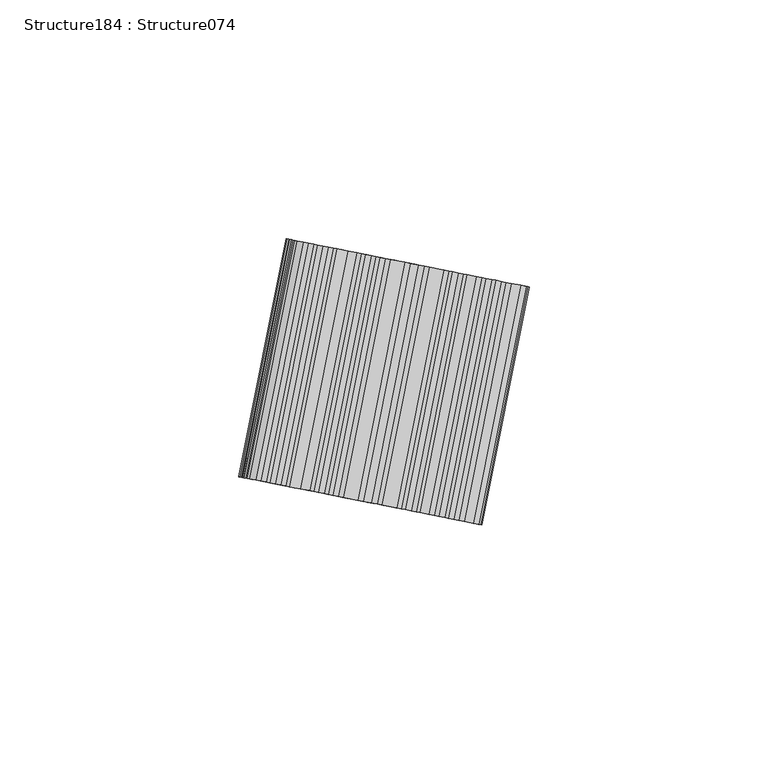
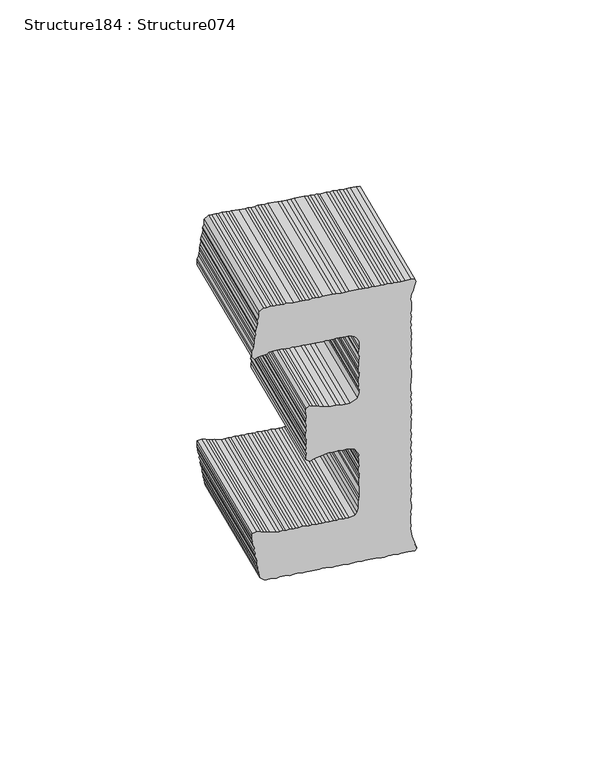
"""IFC4 building model written with IfcOpenShell, lengths in millimetres: proxy geometry, Structure184 : Structure074."""

import ifcopenshell
import ifcopenshell.guid

model = None  # the IFC model being written
_history = None  # IfcOwnerHistory: only IFC2X3 demands one
_inside = {}  # id of a spatial element -> (the spatial element, [elements in it])
_under = {}  # id of a project, library or spatial element -> (it, [spatial elements below it])
_declared = {}  # id of a project -> (the project, [libraries it declares])
_typed = {}  # id of a type object -> (the type object, [elements of that type])
_made_of = {}  # id of a material, layer set ... -> (it, [elements and type objects made of it])


def new_model(schema):
    """Start an empty IFC model of exactly this schema.

    Asked for "IFC4X3", IfcOpenShell would pick the latest addendum, in which some entities
    have other attributes; the version numbers below select the first issue.
    IFC2X3 requires an IfcOwnerHistory on every rooted entity: one is made here for all.
    """
    global model, _history
    if schema == "IFC4X3":
        model = ifcopenshell.file(schema_version=(4, 3, 0, 0))
    else:
        model = ifcopenshell.file(schema=schema)
    _inside.clear()
    _under.clear()
    _declared.clear()
    _typed.clear()
    _made_of.clear()
    _history = None
    if model.schema == "IFC2X3":
        org = make("IfcOrganization", Name="unknown")
        user = make(
            "IfcPersonAndOrganization",
            ThePerson=make("IfcPerson", FamilyName="unknown"),
            TheOrganization=org,
        )
        app = make(
            "IfcApplication",
            ApplicationDeveloper=org,
            Version="unknown",
            ApplicationFullName="unknown",
            ApplicationIdentifier="unknown",
        )
        _history = make(
            "IfcOwnerHistory",
            OwningUser=user,
            OwningApplication=app,
            ChangeAction="ADDED",
            CreationDate=0,
        )
    return model


def make(cls, **values):
    """One entity of the class cls with the attributes given. An attribute that is None is left unset."""
    return model.create_entity(
        cls, **{name: value for name, value in values.items() if value is not None}
    )


def rooted(cls, **values):
    """An entity with a GlobalId (a new one), such as an element, a storey or a relation."""
    return make(cls, GlobalId=ifcopenshell.guid.new(), OwnerHistory=_history, **values)


def si_unit(unit_type, name, prefix=None):
    """IfcSIUnit, for example si_unit("LENGTHUNIT", "METRE", prefix="MILLI")."""
    return make("IfcSIUnit", UnitType=unit_type, Prefix=prefix, Name=name)


def assignment(units):
    """IfcUnitAssignment: the units of a project."""
    return None if units is None else make("IfcUnitAssignment", Units=units)


def point(xyz):
    """IfcCartesianPoint."""
    return None if xyz is None else make("IfcCartesianPoint", Coordinates=xyz)


def direction(xyz):
    """IfcDirection."""
    return None if xyz is None else make("IfcDirection", DirectionRatios=xyz)


def frame(location, z_axis=None, x_axis=None):
    """IfcAxis2Placement3D, a coordinate frame: its origin and axes. An axis left out is left unset."""
    return make(
        "IfcAxis2Placement3D",
        Location=point(location),
        Axis=direction(z_axis),
        RefDirection=direction(x_axis),
    )


def origin():
    """The frame at (0, 0, 0) with its axes left unset."""
    return frame((0.0, 0.0, 0.0))


def place(relative_to, where):
    """IfcLocalPlacement: puts the frame where relative to a parent placement (None: the world)."""
    return make(
        "IfcLocalPlacement", PlacementRelTo=relative_to, RelativePlacement=where
    )


def context(
    kind, dimensions, precision=None, world=None, true_north=None, identifier=None
):
    """IfcGeometricRepresentationContext, for example the 3D "Model" context."""
    return make(
        "IfcGeometricRepresentationContext",
        ContextIdentifier=identifier,
        ContextType=kind,
        CoordinateSpaceDimension=dimensions,
        Precision=precision,
        WorldCoordinateSystem=world,
        TrueNorth=true_north,
    )


def project(units=None, contexts=None):
    """IfcProject with its units and contexts."""
    return rooted(
        "IfcProject",
        Name="project",
        RepresentationContexts=contexts,
        UnitsInContext=assignment(units),
    )


def spatial(cls, under=None, at=None, **own):
    """A site, building, storey or space (cls), placed at a placement, below another one or the project."""
    s = rooted(cls, ObjectPlacement=at, **own)
    if under is not None:
        _under.setdefault(under.id(), (under, []))[1].append(s)
    return s


def polyline(points):
    """IfcPolyline through the points."""
    return make("IfcPolyline", Points=[point(p) for p in points])


def outline(outer, holes=None, kind="AREA"):
    """IfcArbitraryClosedProfileDef: a profile drawn as a closed curve; with holes, ...WithVoids."""
    if holes is None:
        return make("IfcArbitraryClosedProfileDef", ProfileType=kind, OuterCurve=outer)
    return make(
        "IfcArbitraryProfileDefWithVoids",
        ProfileType=kind,
        OuterCurve=outer,
        InnerCurves=holes,
    )


def extrude(swept, where, along, depth):
    """IfcExtrudedAreaSolid: the profile swept, set in the frame where, extruded along a direction by depth."""
    return make(
        "IfcExtrudedAreaSolid",
        SweptArea=swept,
        Position=where,
        ExtrudedDirection=direction(along),
        Depth=depth,
    )


def shape(context_of_items, identifier, shape_type, items):
    """IfcShapeRepresentation: the items that make up one representation, for example the "Body"."""
    return make(
        "IfcShapeRepresentation",
        ContextOfItems=context_of_items,
        RepresentationIdentifier=identifier,
        RepresentationType=shape_type,
        Items=items,
    )


def source(mapping_origin, context_of_items, identifier, shape_type, items):
    """IfcRepresentationMap: a shape defined once, which mapped items show again and again."""
    return make(
        "IfcRepresentationMap",
        MappingOrigin=mapping_origin,
        MappedRepresentation=shape(context_of_items, identifier, shape_type, items),
    )


def transform(
    local_origin,
    x_axis=None,
    y_axis=None,
    z_axis=None,
    scale=None,
    scale2=None,
    scale3=None,
    uniform=True,
):
    """IfcCartesianTransformationOperator3D, or its non-uniform kind. x_axis, y_axis, z_axis: its Axis1, 2, 3."""
    if uniform:
        return make(
            "IfcCartesianTransformationOperator3D",
            Axis1=direction(x_axis),
            Axis2=direction(y_axis),
            LocalOrigin=point(local_origin),
            Scale=scale,
            Axis3=direction(z_axis),
        )
    return make(
        "IfcCartesianTransformationOperator3DnonUniform",
        Axis1=direction(x_axis),
        Axis2=direction(y_axis),
        LocalOrigin=point(local_origin),
        Scale=scale,
        Axis3=direction(z_axis),
        Scale2=scale2,
        Scale3=scale3,
    )


def mapped(mapping_source, mapping_target):
    """IfcMappedItem: shows the shape of a source again, moved by a transform."""
    return make(
        "IfcMappedItem", MappingSource=mapping_source, MappingTarget=mapping_target
    )


def made_of(thing, what):
    """Note that an element or type object is made of a material, layer set ...; save() writes the relation."""
    if what is not None:
        _made_of.setdefault(what.id(), (what, []))[1].append(thing)
    return thing


def element(
    cls,
    number,
    at=None,
    inside=None,
    cuts=None,
    type_object=None,
    material=None,
    context=None,
    identifier="Body",
    shape_type=None,
    held_by="IfcProductDefinitionShape",
    body=None,
    shapes=None,
    **own,
):
    """One element of the class cls, such as IfcWall. Its Tag is "e" and its number.

    at: its placement. inside: the storey or other place that contains it. cuts: it is an
    opening in that element (IfcRelVoidsElement). A single representation is given by context,
    identifier, shape_type and body (its items); several are given by shapes. held_by: the class
    of the entity that holds the representations. save() writes the other relations.
    """
    e = rooted(cls, Tag="e%d" % number, ObjectPlacement=at, **own)
    if body is not None:
        shapes = [shape(context, identifier, shape_type, body)]
    if shapes is not None:
        e.Representation = make(held_by, Representations=shapes)
    if inside is not None:
        _inside.setdefault(inside.id(), (inside, []))[1].append(e)
    if cuts is not None:
        rooted(
            "IfcRelVoidsElement", RelatingBuildingElement=cuts, RelatedOpeningElement=e
        )
    if type_object is not None:
        _typed.setdefault(type_object.id(), (type_object, []))[1].append(e)
    return made_of(e, material)


def aggregate(whole, parts):
    """IfcRelAggregates: a whole, such as a stair, and the parts it consists of."""
    return rooted("IfcRelAggregates", RelatingObject=whole, RelatedObjects=parts)


def save(model, path):
    """Write the relations noted so far, then the file.

    IfcRelAggregates (storeys below a building ...), IfcRelContainedInSpatialStructure (elements
    in a storey), IfcRelDefinesByType, IfcRelAssociatesMaterial and IfcRelDeclares: one each for
    every whole, place, type object, material and project.
    """
    for whole, parts in _under.values():
        aggregate(whole, parts)
    for where, things in _inside.values():
        rooted(
            "IfcRelContainedInSpatialStructure",
            RelatedElements=things,
            RelatingStructure=where,
        )
    for kind, things in _typed.values():
        rooted("IfcRelDefinesByType", RelatedObjects=things, RelatingType=kind)
    for what, things in _made_of.values():
        rooted("IfcRelAssociatesMaterial", RelatedObjects=things, RelatingMaterial=what)
    for by, libraries in _declared.values():
        rooted("IfcRelDeclares", RelatingContext=by, RelatedDefinitions=libraries)
    model.write(path)


def structure184_structure074_331aa3b6(model_context):
    return source(origin(), model_context, "Body", "SweptSolid", [
        extrude(outline(polyline([(1.48162, 0.0), (2.2572372, -0.2724072), (3.0991634, -1.0956216), (4.9019403, -2.1639485), (5.4589513, -2.9293375), (7.3048622, -4.363736), (8.0818521, -4.6349566), (9.0300726, -5.5353617), (9.7680435, -6.2777957), (10.5884484, -6.9153062), (11.4674269, -7.2657789), (12.1278313, -8.1115116), (13.0315131, -8.6447535), (15.4930086, -10.5575032), (16.0253163, -11.140123), (17.6686547, -12.4171089), (18.7521725, -12.9265225), (19.3904936, -13.5861146), (20.2123032, -14.2247167), (21.0525437, -15.0466212), (21.7502814, -15.4198305), (22.753051, -16.0354777), (23.4711862, -16.5935177), (25.1576587, -18.2365751), (25.9576659, -18.6892549), (26.6956368, -19.4316889), (29.8766724, -21.9035703), (30.8579205, -22.3335135), (31.6783254, -22.9710239), (32.3384489, -23.8165383), (33.1384561, -24.2692181), (33.8781127, -25.012962), (34.9840861, -25.7033983), (35.6203492, -26.3667985), (37.2636876, -27.6437844), (38.2676723, -28.2549685), (39.0894819, -28.8935705), (38.9651916, -30.1100787), (37.6526818, -30.742572), (36.993088, -31.3768362), (35.9689867, -32.0626598), (35.0198928, -32.6449986), (33.7000538, -33.9224837), (32.9604919, -34.6631371), (32.347309, -35.6633155), (31.6837244, -36.3061945), (30.4067385, -37.9495329), (29.873026, -38.8474416), (29.1334642, -39.5880949), (28.7015221, -40.5655367), (27.9825762, -41.4907398), (27.3251674, -42.1262514), (26.5015503, -42.9750746), (25.8883673, -43.9752529), (25.4288228, -44.7771356), (24.6908519, -45.5163216), (24.1555485, -46.4156976), (23.3934684, -46.9748293), (22.8595376, -47.8730188), (22.1429933, -48.7951314), (21.4805003, -49.4366057), (20.8432082, -50.2567296), (20.2300253, -51.2569079), (19.4880619, -52.0006518), (18.9530394, -52.9002463), (18.2905464, -53.5417206), (17.7782606, -54.6225558), (16.9608192, -55.4640115), (16.3764867, -56.0049019), (15.944763, -56.9820627), (15.0213404, -57.7488241), (14.486318, -58.6484185), (13.8730723, -59.6480975), (13.1902444, -60.1052404), (12.5733499, -61.110195), (12.1210101, -61.9028061), (11.1943126, -62.6737819), (10.6606001, -63.5716906), (9.3860159, -65.2119384), (8.7701503, -66.2149889), (8.0862308, -66.6735366), (7.4933828, -67.8580463), (6.9377444, -68.5730909), (6.1144083, -69.4221325), (5.5801964, -70.3201037), (4.7425757, -70.9764477), (4.4645531, -71.7558122), (3.5435321, -72.5194831), (3.0301545, -73.6017232), (2.1888223, -74.2628435), (0.9118364, -75.9061818), (0.4560662, -76.7037876), (-0.1801343, -77.5225066), (-0.6359673, -78.3196131), (-1.9943886, -80.0677497), (-2.9140996, -80.8297348), (-4.0071621, -82.4474645), (-4.8283776, -83.293197), (-5.7399809, -84.8879092), (-6.5572039, -85.7290839), (-7.0946906, -86.6312695), (-7.9123503, -87.4730061), (-8.5494241, -88.2928491), (-8.9297165, -88.9927431), (-9.6689973, -89.7336149), (-10.206484, -90.6358005), (-11.8416478, -92.3184934), (-12.1172688, -93.0947674), (-12.9575094, -93.7544829), (-13.6521278, -94.8594595), (-14.0300185, -95.5562629), (-14.9534411, -96.3230244), (-15.4646354, -97.4024548), (-17.2199724, -99.6613778), (-18.1394652, -100.4230819), (-19.05478, -102.0225704), (-19.2578233, -103.3410046), (-19.8695388, -104.3427738), (-20.3033511, -105.3255215), (-20.5537392, -106.2827232), (-21.4192127, -106.761511), (-22.4259747, -106.1504218), (-23.9642339, -104.9550896), (-24.8064733, -104.1293787), (-25.6263162, -103.492305), (-26.6316735, -102.8823073), (-27.1645754, -102.2969728), (-28.3531724, -101.7059054), (-28.9096214, -100.9409531), (-29.9152597, -100.3307372), (-31.3716789, -99.0277668), (-32.1483878, -98.7567645), (-32.8090732, -97.9108135), (-33.9945797, -97.3221476), (-34.5322847, -96.7429942), (-35.4302882, -96.2065043), (-37.8937505, -94.2922263), (-38.6354328, -93.5545686), (-39.5782562, -92.6506971), (-40.9952206, -91.7208527), (-41.9968985, -91.1038007), (-44.458956, -89.1906143), (-45.1190795, -88.3450999), (-46.2028783, -87.8354679), (-46.9207325, -87.2776462), (-47.4771815, -86.512694), (-48.5046544, -85.7142776), (-49.3057533, -85.2630027), (-49.9423296, -84.597106), (-51.478622, -83.4033022), (-53.4873429, -82.1749426), (-53.9403985, -81.4903341), (-54.9230514, -81.0592993), (-55.8471308, -80.3412267), (-56.6910828, -79.5240985), (-57.3851089, -79.1461129), (-58.2304657, -78.3278931), (-59.0522754, -77.6892909), (-59.437277, -76.0675653), (-58.3214154, -74.6315759), (-57.9340122, -73.2869709), (-57.2742018, -72.6483689), (-56.8965294, -71.9518463), (-56.56848, -70.8941234), (-55.9773177, -69.7083038), (-55.3156032, -69.0707307), (-54.9631637, -68.1932805), (-54.5269176, -67.2097203), (-53.9725892, -66.4963614), (-53.3575987, -65.4903778), (-52.9805187, -64.7951975), (-52.5729988, -63.6352049), (-52.1137353, -62.8331038), (-51.4766615, -62.0132609), (-50.3029741, -61.7739762), (-50.10932, -62.581905), (-49.2688612, -63.4035286), (-48.6049635, -64.2447659), (-47.8648075, -64.9884473), (-47.6716526, -65.7964387), (-45.9830917, -67.4339092), (-44.3397534, -68.710895), (-43.4642681, -69.0658631), (-42.5421555, -69.7824074), (-41.8782578, -70.6236447), (-40.8988172, -71.0593933), (-40.1809629, -71.617215), (-39.518751, -72.4571423), (-38.4143042, -73.1536021), (-35.9525276, -75.0665702), (-35.0517468, -75.6029653), (-34.3338925, -76.160787), (-33.5694109, -77.0801848), (-32.6936448, -77.4353712), (-31.7454241, -78.3357763), (-31.2082183, -78.9149923), (-29.5679706, -80.1895766), (-28.667782, -80.7273139), (-27.8226435, -81.5458146), (-26.091727, -82.0716378), (-24.9148275, -81.8276393), (-23.6088048, -81.2040741), (-22.1744063, -79.3581631), (-21.7967338, -78.6616407), (-21.185174, -77.6606517), (-20.2581634, -76.8921723), (-19.3224509, -75.4775145), (-18.6067799, -74.5565258), (-17.99522, -73.5555368), (-17.4334685, -72.8326253), (-16.5920415, -72.1742824), (-16.0364031, -71.4592377), (-15.5207188, -70.3711298), (-14.9663904, -69.6577709), (-14.14377, -68.8131299), (-13.6101523, -67.9124439), (-12.7682887, -67.253539), (-12.2864443, -66.6334591), (-11.6033033, -64.6971925), (-12.7339798, -62.3423672), (-13.6792996, -61.4388089), (-15.1169749, -60.3216373), (-16.3013897, -59.7315667), (-17.9444471, -58.4547991), (-19.6194081, -57.6493667), (-20.8856037, -57.1593197), (-21.7611517, -56.8038523), (-22.8446695, -56.2944386), (-23.9836434, -56.0645715), (-24.2452299, -54.7050245), (-23.8705513, -54.0129348), (-22.3881206, -52.5296916), (-21.6973712, -51.4262148), (-21.3167979, -50.726539), (-20.4777725, -50.0712867), (-19.7844032, -48.9644382), (-19.2020966, -48.429634), (-18.6883772, -47.3440548), (-17.9731429, -46.4236279), (-17.127786, -45.7602277), (-16.4907122, -44.9403848), (-16.0331344, -44.1369737), (-15.3748506, -43.5043953), (-14.865061, -42.4238733), (-14.0978647, -41.8610569), (-13.5658379, -40.9618384), (-12.8492936, -40.0397258), (-11.3397581, -40.2177813), (-10.9453387, -41.1889281), (-10.3872361, -41.9529122), (-9.5147744, -42.9508106), (-8.936523, -43.9016852), (-7.6375486, -45.40495), (-6.8375413, -45.8576298), (-5.8925025, -46.7609697), (-5.3556082, -47.3417462), (-4.1701017, -47.9304121), (-3.5344004, -48.5933756), (-2.6089163, -49.3125398), (-0.8759114, -49.832776), (1.5023395, -48.8888325), (1.7787391, -48.1086572), (2.6760267, -47.1679277), (3.3133188, -46.3478038), (3.9768407, -45.7044254), (4.325506, -44.8312522), (4.9649814, -44.0083187), (5.8895904, -43.2429298), (6.5268826, -42.4228059), (6.9034634, -41.7276882), (8.0985772, -40.1897101), (8.9184201, -39.3451638), (10.8324798, -36.8819825), (11.2090607, -36.1868648), (11.8208388, -35.185595), (13.1770768, -33.4402679), (13.7251051, -31.8883767), (13.7916325, -30.9572831), (12.5728444, -29.347348), (11.6711295, -28.8156345), (11.216388, -28.1297161), (10.0308816, -27.5410502), (9.5758593, -26.8549135), (8.6753594, -26.3187367), (7.8308132, -25.4988938), (6.6439019, -24.9091362), (5.9832165, -24.0631853), (5.0841214, -23.5281001), (4.4438335, -22.8669798), (3.3620016, -22.3588761), (2.8035858, -21.5923956), (2.0064793, -21.1365626), (1.000809, -20.5240685), (0.1361461, -19.5196132), (-0.6612412, -19.063562), (-1.4032368, -18.3234078), (-2.2824962, -17.9727167), (-3.1457542, -16.9693531), (-3.9224631, -16.6983507), (-4.5831485, -15.8523998), (-5.4046772, -15.214016), (-7.3669552, -14.3538486), (-8.2671436, -13.8161113), (-9.1459038, -13.4653575), (-10.1011405, -13.2124408), (-11.2864609, -12.6212158), (-12.2547033, -11.5389758), (-11.4562869, -10.511503), (-10.8200864, -9.6927839), (-10.1364479, -9.2340179), (-9.2370718, -8.2877014), (-8.2901611, -7.7081721), (-7.8362949, -6.9095374), (-6.8680525, -6.5101574), (-6.3302848, -5.6081901), (-5.40945, -4.8470783), (-4.5434772, -4.3682278), (-3.7463708, -3.3424408), (-2.9842908, -2.7833092), (-2.4264691, -2.065455), (-1.4788426, -1.4815252), (-0.5802451, -0.5391099), (0.0, 0.0), (1.48162, 0.0)])), frame((-1908.6751886, 234847.2710242, 387.6985279), z_axis=(0.19466222296394123, 0.9808703374813293, 0.0), x_axis=(0.7745184631426425, -0.15370990435811277, -0.6135914076593472)), (0.0, 0.0, 1.0), 50.8),
    ])


if __name__ == "__main__":
    model = new_model("IFC4")
    model_context = context("Model", 3, world=origin())
    ifc_project = project(units=[si_unit("LENGTHUNIT", "METRE", prefix="MILLI")], contexts=[model_context])
    site = spatial("IfcSite", under=ifc_project)
    building = spatial("IfcBuilding", under=site)
    placement = place(None, origin())
    structure184_structure074_shape = structure184_structure074_331aa3b6(model_context)
    element("IfcBuildingElementProxy", 1, Name="Structure184 : Structure074", ObjectType="Structure184 : Structure074", at=placement, inside=building, context=model_context, shape_type="MappedRepresentation", body=[
        mapped(structure184_structure074_shape, transform((0.0, 0.0, 0.0), x_axis=(1.0, 0.0, 0.0), y_axis=(0.0, 1.0, 0.0), z_axis=(0.0, 0.0, 1.0))),
    ])
    save(model, "model.ifc")

# Revit data of these elements
# Type "Structure184 : Structure074"
#   NameOverride = "Structure074"
# Element 1 (IfcBuildingElementProxy, "Structure184 : Structure074")
#   Materials on its faces: "BRUSHED ALUMINUM LETTERING"
# Materials
#   "BRUSHED ALUMINUM LETTERING": class "Unassigned", colour RGB 169 181 186, transparency 0, Cost = 0
